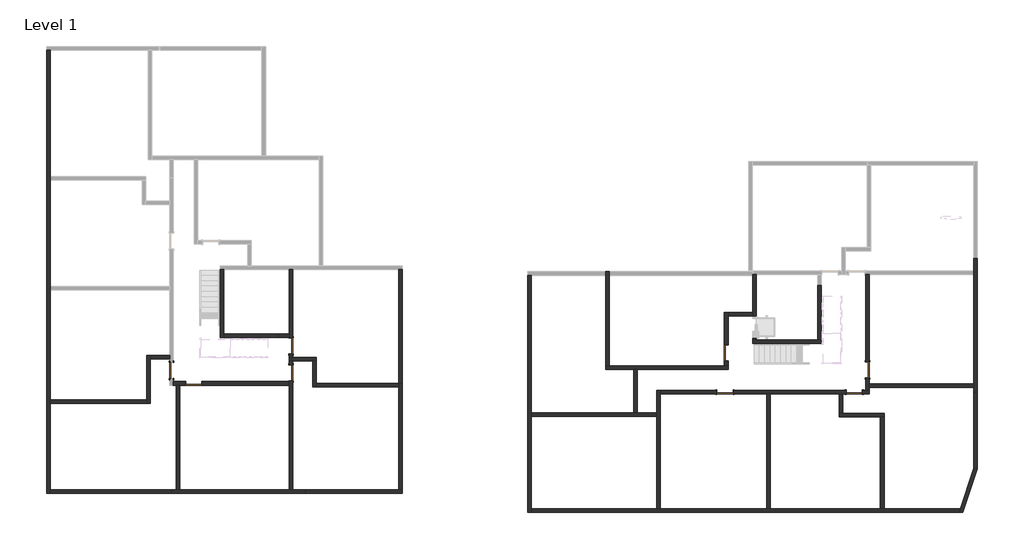
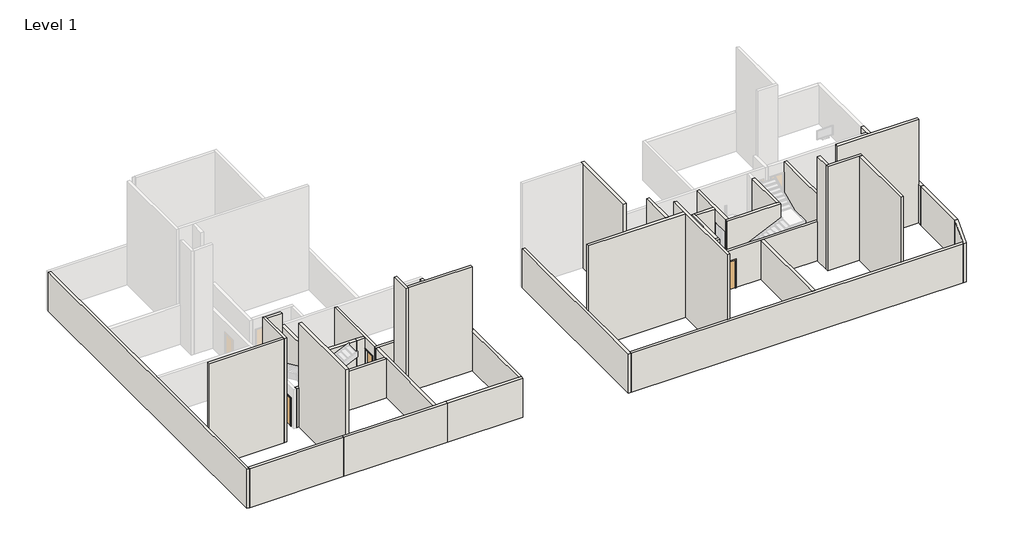
# One storey, part 1 of 2: 41 walls, 8 doors.
# Revit data of these elements (continued)
# Room, not placed, phase "New Construction", upper offset 0 cm, lower offset 0 cm (continued)
#   Name = "Room"
# Room, not placed, phase "New Construction", upper offset 0 cm, lower offset 0 cm
#   Number = "128"
#   Name = "Room"
# Room, not placed, phase "New Construction", upper offset 0 cm, lower offset 0 cm
#   Number = "129"
#   Name = "Room"
# Room, not placed, phase "New Construction", upper offset 0 cm, lower offset 0 cm
#   Number = "91"
#   Name = "Room"
# Room at (-20321.225, 11202.195) mm, phase "New Construction", upper level "Level 1", upper offset 243.84 cm, lower offset 0 cm
#   Number = "130"
#   Name = "Room"
# Room at (-5594.466, -7580.79) mm, phase "New Construction", upper level "Level 1", upper offset 243.84 cm, lower offset 0 cm
#   Number = "131"
#   Name = "Room"
# Room at (-4954.966, -1430.614) mm, phase "New Construction", upper level "Level 1", upper offset 243.84 cm, lower offset 0 cm
#   Number = "132"
#   Name = "Room"
# Room at (-12237.947, 10302.814) mm, phase "New Construction", upper level "Level 1", upper offset 243.84 cm, lower offset 0 cm
#   Number = "133"
#   Name = "Room"
# Room, not placed, phase "New Construction", upper offset 0 cm, lower offset 0 cm
#   Number = ""
#   Name = ""
# Room, not placed, phase "New Construction", upper offset 0 cm, lower offset 0 cm
#   Number = "70"
#   Name = "Room"
# Room, not placed, phase "New Construction", upper offset 0 cm, lower offset 0 cm
#   Number = "71"
#   Name = "Room"
# Room, not placed, phase "New Construction", upper offset 0 cm, lower offset 0 cm
#   Number = "92"
#   Name = "Room"
# Room, not placed, phase "New Construction", upper offset 0 cm, lower offset 0 cm
#   Number = ""
#   Name = ""
# Room, not placed, phase "New Construction", upper offset 0 cm, lower offset 0 cm
#   Number = ""
#   Name = ""
# Room, not placed, phase "New Construction", upper offset 0 cm, lower offset 0 cm
#   Number = "37"
#   Name = "Room"
# Room, not placed, phase "New Construction", upper offset 0 cm, lower offset 0 cm
#   Number = ""
#   Name = "Banyo"
# Room, not placed, phase "New Construction", upper offset 0 cm, lower offset 0 cm
#   Number = ""
#   Name = ""
# Room, not placed, phase "New Construction", upper offset 0 cm, lower offset 0 cm
#   Number = ""
#   Name = "Yatak Odası"
# Room, not placed, phase "New Construction", upper offset 0 cm, lower offset 0 cm
#   Number = "39"
#   Name = "Room"
# Room, not placed, phase "New Construction", upper offset 0 cm, lower offset 0 cm
#   Number = ""
#   Name = "Salon-Mutfak"
# Area at (-11214.009, 13625.616) mm, upper offset 243.84 cm, lower offset 0 cm
#   Number = "9"
#   Name = "Area"
# Room, not placed, phase "New Construction", upper offset 0 cm, lower offset 0 cm
#   Number = "134"
#   Name = "Room"
# Room at (-19334.034, -2481.955) mm, phase "New Construction", upper level "Level 1", upper offset 243.84 cm, lower offset 0 cm
#   Number = "135"
#   Name = "Room"
# Room, not placed, phase "New Construction", upper offset 0 cm, lower offset 0 cm
#   Number = "40"
#   Name = "Room"
# Room, not placed, phase "New Construction", upper offset 0 cm, lower offset 0 cm
#   Number = "41"
#   Name = "Room"
# Area, not placed, upper offset 0 cm, lower offset 0 cm
#   Number = "8"
#   Name = "Dere Parsel Toplam Alan"
# Room, not placed, phase "New Construction", upper offset 0 cm, lower offset 0 cm
#   Number = "108"
#   Name = "ASANSÖR"
# Room, not placed, phase "New Construction", upper offset 0 cm, lower offset 0 cm
#   Number = "89"
#   Name = "Room"
# Room, not placed, phase "New Construction", upper offset 0 cm, lower offset 0 cm
#   Number = "19"
#   Name = "Room"
# Room, not placed, phase "New Construction", upper offset 0 cm, lower offset 0 cm
#   Number = ""
#   Name = ""
# Room, not placed, phase "New Construction", upper offset 0 cm, lower offset 0 cm
#   Number = "21"
#   Name = "Room"
# Room, not placed, phase "New Construction", upper offset 0 cm, lower offset 0 cm
#   Number = "22"
#   Name = "Room"
# Room, not placed, phase "New Construction", upper offset 0 cm, lower offset 0 cm
#   Number = "23"
#   Name = "Room"
# Room, not placed, phase "New Construction", upper offset 0 cm, lower offset 0 cm
#   Number = "24"
#   Name = "Room"
# Room, not placed, phase "New Construction", upper offset 0 cm, lower offset 0 cm
#   Number = "25"
#   Name = "Room"
# Room, not placed, phase "New Construction", upper offset 0 cm, lower offset 0 cm
#   Number = "64"
#   Name = "Room"
# Room, not placed, phase "New Construction", upper offset 0 cm, lower offset 0 cm
#   Number = "65"
#   Name = "Room"
# Room, not placed, phase "New Construction", upper offset 0 cm, lower offset 0 cm
#   Number = "66"
#   Name = "Room"
# Room, not placed, phase "New Construction", upper offset 0 cm, lower offset 0 cm
#   Number = ""
#   Name = ""
# Room, not placed, phase "New Construction", upper offset 0 cm, lower offset 0 cm
#   Number = "27"
#   Name = "Room"
# Room, not placed, phase "New Construction", upper offset 0 cm, lower offset 0 cm
#   Number = "42"
#   Name = "Room"
# Area, not placed, upper offset 0 cm, lower offset 0 cm
#   Number = "2"
#   Name = "Area"
# Room, not placed, phase "New Construction", upper offset 0 cm, lower offset 0 cm
#   Number = "43"
#   Name = "Room"
# Room, not placed, phase "New Construction", upper offset 0 cm, lower offset 0 cm
#   Number = ""
#   Name = ""
# Room, not placed, phase "New Construction", upper offset 0 cm, lower offset 0 cm
#   Number = "94"
#   Name = "Room"
# Room, not placed, phase "New Construction", upper offset 0 cm, lower offset 0 cm
#   Number = ""
#   Name = ""
# Room at (-18935.383, 3898.657) mm, phase "New Construction", upper level "Level 1", upper offset 243.84 cm, lower offset 0 cm
#   Number = "136"
#   Name = "Room"
# Room, not placed, phase "New Construction", upper offset 0 cm, lower offset 0 cm
#   Number = "1"
#   Name = "Room"
# Area, not placed, upper offset 0 cm, lower offset 0 cm
#   Number = "3"
#   Name = "Area"
# Room, not placed, phase "New Construction", upper offset 0 cm, lower offset 0 cm
#   Number = "7"
#   Name = "Room"
# Room, not placed, phase "New Construction", upper offset 0 cm, lower offset 0 cm
#   Number = "8"
#   Name = "Room"
# Room, not placed, phase "New Construction", upper offset 0 cm, lower offset 0 cm
#   Number = "2"
#   Name = "Room"
# Room, not placed, phase "New Construction", upper offset 0 cm, lower offset 0 cm
#   Number = "46"
#   Name = "Room"
# Room, not placed, phase "New Construction", upper offset 0 cm, lower offset 0 cm
#   Number = "3"
#   Name = "Room"
# Room, not placed, phase "New Construction", upper offset 0 cm, lower offset 0 cm
#   Number = ""
#   Name = ""
# Room, not placed, phase "New Construction", upper offset 0 cm, lower offset 0 cm
#   Number = "4"
#   Name = "Room"
# Area, not placed, upper offset 0 cm, lower offset 0 cm
#   Number = "1"
#   Name = "Area"
# Room, not placed, phase "New Construction", upper offset 0 cm, lower offset 0 cm
#   Number = ""
#   Name = ""
# Room, not placed, phase "New Construction", upper offset 0 cm, lower offset 0 cm
#   Number = "29"
#   Name = "Room"
# Area, not placed, upper offset 0 cm, lower offset 0 cm
#   Number = "7"
#   Name = "Dere Parsel Toplam Alan"
# Room, not placed, phase "New Construction", upper offset 0 cm, lower offset 0 cm
#   Number = "95"
#   Name = "ASANSÖR"
# Room, not placed, phase "New Construction", upper offset 0 cm, lower offset 0 cm
#   Number = "96"
#   Name = "Room"
# Room, not placed, phase "New Construction", upper offset 0 cm, lower offset 0 cm
#   Number = "97"
#   Name = "7"
# Room, not placed, phase "New Construction", upper offset 0 cm, lower offset 0 cm
#   Number = "98"
#   Name = "8"
# Room, not placed, phase "New Construction", upper offset 0 cm, lower offset 0 cm
#   Number = "99"
#   Name = "9"
# Room, not placed, phase "New Construction", upper offset 0 cm, lower offset 0 cm
#   Number = "100"
#   Name = "1"
# Room, not placed, phase "New Construction", upper offset 0 cm, lower offset 0 cm
#   Number = "101"
#   Name = "5"
# Room, not placed, phase "New Construction", upper offset 0 cm, lower offset 0 cm
#   Number = "102"
#   Name = "2"
# Room, not placed, phase "New Construction", upper offset 0 cm, lower offset 0 cm
#   Number = "103"
#   Name = "4"
# Room, not placed, phase "New Construction", upper offset 0 cm, lower offset 0 cm
#   Number = "104"
#   Name = "3"
# Room, not placed, phase "New Construction", upper offset 0 cm, lower offset 0 cm
#   Number = "105"
#   Name = "6"
